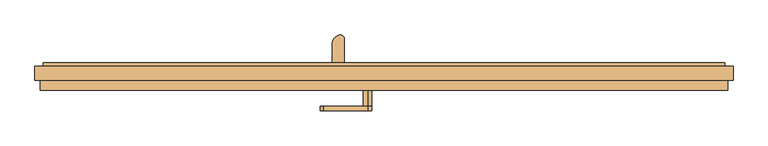
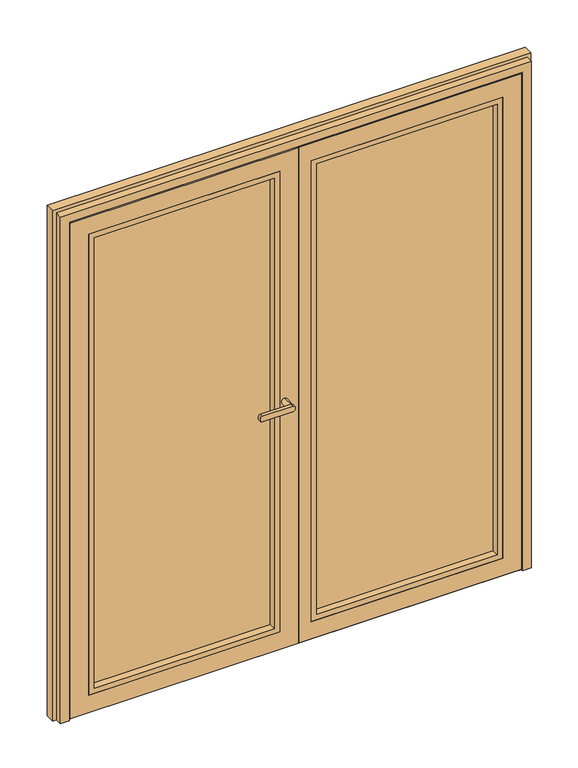
"""IFC4 building model written with IfcOpenShell, lengths in millimetres: door geometry, Schueco_FWS_ADS-75-HD-HI_inw_Family-02 : FWS SI insert unit."""

from ifc_helpers import new_model, si_unit, point, frame, frame_2d, origin, place, context, project, spatial, polyline, circle_curve, ellipse_curve, trimmed, segment, composite_curve, outline, extrude, faceted_brep, source, transform, mapped, element, save
from ifc_brep_helpers import plane_surface, cylinder_surface, extruded_surface, advanced_brep


def door_6b0dbaab(model_context):
    return source(origin(), model_context, "Body", "SolidModel", [
        faceted_brep([(900.0, -57.5000065, 8.0), (900.0, -57.5000065, 2100.0), (900.0, -66.0002823, 2100.0), (900.0, -66.0002823, 8.0), (15.0, -66.0002823, 8.0), (15.0, -57.5000065, 8.0), (15.0, -57.5000065, 23.0), (885.0, -57.5000065, 23.0), (885.0, -57.5000065, 2085.0), (15.0, -57.5000065, 2085.0), (15.0, -57.5000065, 2100.0), (15.0, -66.0002823, 2100.0), (63.0, -66.0002823, 81.0), (63.0, -66.0002823, 2027.0), (827.0, -66.0002823, 2027.0), (827.0, -66.0002823, 81.0), (827.0, 0.4997603, 2027.0), (827.0, 0.4997603, 81.0), (63.0, 0.4997603, 81.0), (63.0, 0.4997603, 2027.0), (88.0, 0.4997603, 106.0), (88.0, 0.4997603, 2002.0), (802.0, 0.4997603, 2002.0), (802.0, 0.4997603, 106.0), (802.0, 8.9997177, 2002.0), (802.0, 8.9997177, 106.0), (88.0, 8.9997177, 106.0), (88.0, 8.9997177, 2002.0), (875.0, 8.9997177, 33.0), (-10.0, 8.9997177, 33.0), (-10.0, 8.9997177, 2075.0), (875.0, 8.9997177, 2075.0), (875.0, 0.4997603, 2075.0), (875.0, 0.4997603, 33.0), (5.0, 0.4997603, 33.0), (-10.0, 0.4997603, 33.0), (5.0, 0.4997603, 23.0), (5.0, 0.4997603, 2075.0), (5.0, 0.4997603, 2085.0), (885.0, 0.4997603, 2085.0), (885.0, 0.4997603, 23.0), (5.0, -57.5000065, 23.0), (5.0, -57.5000065, 2085.0), (-10.0, 0.4997603, 2075.0)], [[[0, 1, 2, 3]], [[3, 4, 5, 0]], [[0, 5, 6, 7, 8, 9, 10, 1]], [[2, 11, 4, 3], [12, 13, 14, 15]], [[15, 14, 16, 17]], [[17, 18, 12, 15]], [[18, 19, 13, 12]], [[17, 16, 19, 18], [20, 21, 22, 23]], [[23, 22, 24, 25]], [[25, 26, 20, 23]], [[26, 27, 21, 20]], [[28, 29, 30, 31], [25, 24, 27, 26]], [[28, 31, 32, 33]], [[33, 34, 35, 29, 28]], [[36, 34, 33, 32, 37, 38, 39, 40]], [[40, 39, 8, 7]], [[7, 6, 41, 36, 40]], [[41, 42, 38, 37, 34, 36]], [[1, 10, 11, 2]], [[19, 16, 14, 13]], [[27, 24, 22, 21]], [[31, 30, 43, 37, 32]], [[42, 9, 8, 39, 38]], [[6, 5, 4, 11, 10, 9]], [[35, 43, 30, 29]], [[35, 34, 37, 43]], [[9, 42, 41, 6]]]),
        extrude(outline(polyline([(81.0, 63.0), (81.0, 827.0), (2027.0, 827.0), (2027.0, 63.0), (81.0, 63.0)]), holes=[polyline([(103.0, 805.0), (103.0, 85.0), (2005.0, 85.0), (2005.0, 805.0), (103.0, 805.0)])]), frame((0.0, -66.0002823, 0.0), z_axis=(0.0, 1.0, 0.0), x_axis=(0.0, 0.0, 1.0)), (0.0, 0.0, 1.0), 28.5000426),
        extrude(outline(polyline([(63.0, -37.5002397), (63.0, 0.4997603), (827.0, 0.4997603), (827.0, -37.5002397), (63.0, -37.5002397)])), frame((0.0, 0.0, 81.0), z_axis=(0.0, 0.0, 1.0), x_axis=(1.0, 0.0, 0.0)), (0.0, 0.0, 1.0), 1946.0),
        extrude(outline(polyline([(875.0, 0.4997603), (-10.0, 0.4997603), (-10.0, 8.9997177), (875.0, 8.9997177), (875.0, 0.4997603)])), frame((0.0, 0.0, 23.0), z_axis=(0.0, 0.0, 1.0), x_axis=(1.0, 0.0, 0.0)), (0.0, 0.0, 1.0), 10.0),
        extrude(outline(composite_curve([segment(polyline([(-141.6673236, 8.9997177), (-141.6673236, 59.1618682)]), True, "CONTINUOUS"), segment(trimmed(circle_curve(frame_2d((-114.4889059, 59.1618682)), 27.1784177), [point((-141.6673236, 59.1618682))], [point((-124.0260015, 84.6120194))], False, "CARTESIAN"), True, "CONTINUOUS"), segment(trimmed(circle_curve(frame_2d((-119.9485005, 73.7310321)), 11.6198924), [point((-124.0260015, 84.6120194))], [point((-108.3286081, 73.7310321))], False, "CARTESIAN"), True, "CONTINUOUS"), segment(polyline([(-108.3286081, 73.7310321), (-108.3286081, 8.9997177), (-141.6673236, 8.9997177)]), True, "CONTINUOUS")], self_intersect=False)), frame((0.0, 0.0, 2043.9340013), z_axis=(0.0, 0.0, 1.0), x_axis=(1.0, 0.0, 0.0)), (0.0, 0.0, 1.0), 4.0),
        extrude(outline(polyline([(-141.6673236, 12.9997177), (-108.3286081, 12.9997177), (-108.3286081, 8.9997177), (-141.6673236, 8.9997177), (-141.6673236, 12.9997177)])), frame((0.0, 0.0, 2013.9340013), z_axis=(0.0, 0.0, 1.0), x_axis=(1.0, 0.0, 0.0)), (0.0, 0.0, 1.0), 30.0),
        extrude(outline(polyline([(-141.6673236, 12.9997177), (-108.3286081, 12.9997177), (-108.3286081, 8.9997177), (-141.6673236, 8.9997177), (-141.6673236, 12.9997177)])), frame((0.0, 0.0, 56.9340013), z_axis=(0.0, 0.0, 1.0), x_axis=(1.0, 0.0, 0.0)), (0.0, 0.0, 1.0), 30.0),
        extrude(outline(composite_curve([segment(polyline([(-141.6673236, 8.9997177), (-141.6673236, 59.1618682)]), True, "CONTINUOUS"), segment(trimmed(circle_curve(frame_2d((-114.4889059, 59.1618682)), 27.1784177), [point((-141.6673236, 59.1618682))], [point((-124.0260015, 84.6120194))], False, "CARTESIAN"), True, "CONTINUOUS"), segment(trimmed(circle_curve(frame_2d((-119.9485005, 73.7310321)), 11.6198924), [point((-124.0260015, 84.6120194))], [point((-108.3286081, 73.7310321))], False, "CARTESIAN"), True, "CONTINUOUS"), segment(polyline([(-108.3286081, 73.7310321), (-108.3286081, 8.9997177), (-141.6673236, 8.9997177)]), True, "CONTINUOUS")], self_intersect=False)), frame((0.0, 0.0, 52.9340013), z_axis=(0.0, 0.0, 1.0), x_axis=(1.0, 0.0, 0.0)), (0.0, 0.0, 1.0), 4.0),
        advanced_brep(
        [(-112.282924, 57.5977179, 2043.9340013), (-137.717076, 72.2821425, 2043.9340013), (-112.282924, 57.5977179, 56.9340013), (-137.717076, 72.2821425, 56.9340013)],
        [
            (0, 1, ellipse_curve(frame((-125.0, 64.9399302, 2043.9340013), z_axis=(0.0, 0.0, 1.0000000000000002), x_axis=(0.5000002582658958, 0.866025254674503, 0.0)), 21.5840887, 14.6844171)),
            (1, 0, ellipse_curve(frame((-125.0, 64.9399302, 2043.9340013), z_axis=(0.0, 0.0, 1.0000000000000002), x_axis=(0.5000002582658958, 0.866025254674503, 0.0)), 21.5840887, 14.6844171)),
            (2, 3, ellipse_curve(frame((-125.0, 64.9399302, 56.9340013), z_axis=(0.0, 0.0, -1.0000000000000002), x_axis=(-0.866025254674503, 0.5000002582658958, 0.0)), 14.6844171, 21.5840887)),
            (3, 2, ellipse_curve(frame((-125.0, 64.9399302, 56.9340013), z_axis=(0.0, 0.0, -1.0000000000000002), x_axis=(-0.866025254674503, 0.5000002582658958, 0.0)), 14.6844171, 21.5840887)),
            (0, 2),
            (3, 1),
        ],
        [
            plane_surface(frame((-137.717076, 72.2821425, 2043.9340013), z_axis=(0.0, 0.0, 1.0000000000000002), x_axis=(0.5000002582658958, 0.866025254674503, 0.0))),
            plane_surface(frame((-137.717076, 72.2821425, 56.9340013), z_axis=(0.0, 0.0, -1.0000000000000002), x_axis=(-0.5000002582658958, -0.866025254674503, 0.0))),
            extruded_surface(trimmed(ellipse_curve(frame((-125.0, 64.9399302, 56.9340013), z_axis=(0.0, 0.0, -1.0000000000000002), x_axis=(-0.866025254674503, 0.5000002582658958, 0.0)), 14.6844171, 21.5840887), [point((-137.717076, 72.2821425, 56.9340013))], [point((-112.282924, 57.5977179, 56.9340013))], True, "CARTESIAN"), (0.0, 0.0, -1987.0), 1987.0),
            extruded_surface(trimmed(ellipse_curve(frame((-125.0, 64.9399302, 56.9340013), z_axis=(0.0, 0.0, -1.0000000000000002), x_axis=(-0.866025254674503, 0.5000002582658958, 0.0)), 14.6844171, 21.5840887), [point((-112.282924, 57.5977179, 56.9340013))], [point((-137.717076, 72.2821425, 56.9340013))], True, "CARTESIAN"), (0.0, 0.0, -1987.0), 1987.0),
        ],
        [
            (0, [[1, 2]]),
            (1, [[3, 4]]),
            (2, [[5, -4, 6, -1]]),
            (3, [[-6, -3, -5, -2]]),
        ],
    ),
        advanced_brep(
        [(-45.0, -122.0002518, 1038.0113692), (-45.0, -122.0002518, 1061.9886308), (-166.6617926, -122.0002518, 1061.9886308), (-166.6617926, -122.0002518, 1038.0113692), (-45.0, -109.5001648, 1061.9886308), (-45.0, -109.5001648, 1038.0113692), (-166.6617926, -109.5001648, 1038.0113692), (-166.6617926, -109.5001648, 1061.9886308), (-45.0, -66.0002823, 1038.0113692), (-45.0, -66.0002823, 1061.9886308)],
        [
            (0, 1, circle_curve(frame((-45.0, -122.0002518, 1050.0), z_axis=(0.0, -1.0, 0.0), x_axis=(0.0, 0.0, 1.0)), 11.9886308)),
            (1, 2),
            (2, 3, ellipse_curve(frame((-166.6617926, -122.0002518, 1050.0), z_axis=(0.0, -1.0, 0.0), x_axis=(0.0, 0.0, -1.0)), 11.9886308, 7.9050795)),
            (3, 0),
            (4, 5, circle_curve(frame((-45.0, -109.5001648, 1050.0), z_axis=(0.0, -1.0, 0.0), x_axis=(0.0, 0.0, 1.0)), 11.9886308)),
            (5, 6),
            (6, 7, ellipse_curve(frame((-166.6617926, -109.5001648, 1050.0), z_axis=(0.0, 1.0, 0.0), x_axis=(0.0, 0.0, -1.0)), 11.9886308, 7.9050795)),
            (7, 4),
            (3, 6),
            (5, 0),
            (2, 7),
            (1, 4),
            (5, 4, circle_curve(frame((-45.0, -109.5001648, 1050.0), z_axis=(0.0, -1.0, 0.0), x_axis=(0.0, 0.0, 1.0)), 11.9886308)),
            (8, 9, circle_curve(frame((-45.0, -66.0002823, 1050.0), z_axis=(0.0, 1.0, 0.0), x_axis=(0.0, 0.0, 1.0)), 11.9886308)),
            (9, 8, circle_curve(frame((-45.0, -66.0002823, 1050.0), z_axis=(0.0, 1.0, 0.0), x_axis=(0.0, 0.0, 1.0)), 11.9886308)),
            (8, 5),
            (4, 9),
        ],
        [
            plane_surface(frame((-166.6617926, -122.0002518, 1038.0113692), z_axis=(0.0, -1.0, 0.0), x_axis=(-1.0, 0.0, 0.0))),
            plane_surface(frame((-166.6617926, -109.5001648, 1038.0113692), z_axis=(0.0, 1.0, 0.0), x_axis=(1.0, 0.0, 0.0))),
            plane_surface(frame((-45.0, -122.0002518, 1038.0113692), z_axis=(0.0, 0.0, -1.0), x_axis=(0.0, 1.0, 0.0))),
            extruded_surface(trimmed(ellipse_curve(frame((-166.6617926, -109.5001648, 1050.0), z_axis=(0.0, 1.0, 0.0), x_axis=(0.0, 0.0, -1.0)), 11.9886308, 7.9050795), [point((-166.6617926, -109.5001648, 1038.0113692))], [point((-166.6617926, -109.5001648, 1061.9886308))], True, "CARTESIAN"), (0.0, 12.500086999999994, 0.0), 12.500086999999994),
            plane_surface(frame((-166.6617926, -122.0002518, 1061.9886308), z_axis=(0.0, 0.0, 1.0), x_axis=(0.0, 1.0, 0.0))),
            cylinder_surface(frame((-45.0, -109.5001648, 1050.0), z_axis=(0.0, -1.0, 0.0), x_axis=(0.0, 0.0, 1.0)), 11.9886308),
            plane_surface(frame((-45.0, -66.0002823, 1061.9886308), z_axis=(0.0, 1.0, 0.0), x_axis=(-1.0, 0.0, 0.0))),
            cylinder_surface(frame((-45.0, -66.0002823, 1050.0), z_axis=(0.0, -1.0, 0.0), x_axis=(0.0, 0.0, 1.0)), 11.9886308),
        ],
        [
            (0, [[1, 2, 3, 4]]),
            (1, [[5, 6, 7, 8]]),
            (2, [[9, -6, 10, -4]]),
            (3, [[11, -7, -9, -3]]),
            (4, [[12, -8, -11, -2]]),
            (5, [[-10, 13, -12, -1]]),
            (6, [[14, 15]]),
            (7, [[16, -5, 17, -14]]),
            (7, [[-17, -13, -16, -15]]),
        ],
    ),
        faceted_brep([(-900.0, -57.5000065, 8.0), (-900.0, -66.0002823, 8.0), (-900.0, -66.0002823, 2100.0), (-900.0, -57.5000065, 2100.0), (10.0, -57.5000065, 8.0), (10.0, -66.0002823, 8.0), (10.0, -57.5000065, 2100.0), (-885.0, -57.5000065, 23.0), (-5.0, -57.5000065, 23.0), (-5.0, -57.5000065, 2085.0), (-885.0, -57.5000065, 2085.0), (10.0, -66.0002823, 2100.0), (-63.0, -66.0002823, 81.0), (-827.0, -66.0002823, 81.0), (-827.0, -66.0002823, 2027.0), (-63.0, -66.0002823, 2027.0), (-827.0, 0.4997603, 81.0), (-827.0, 0.4997603, 2027.0), (-63.0, 0.4997603, 81.0), (-63.0, 0.4997603, 2027.0), (-88.0, 0.4997603, 106.0), (-802.0, 0.4997603, 106.0), (-802.0, 0.4997603, 2002.0), (-88.0, 0.4997603, 2002.0), (-802.0, 8.9997177, 106.0), (-802.0, 8.9997177, 2002.0), (-88.0, 8.9997177, 106.0), (-88.0, 8.9997177, 2002.0), (-15.0, 8.9997177, 2075.0), (-15.0, 8.9997177, 33.0), (-25.0, 8.9997177, 33.0), (-875.0, 8.9997177, 33.0), (-875.0, 8.9997177, 2075.0), (-25.0, 8.9997177, 2075.0), (-875.0, 0.4997603, 33.0), (-875.0, 0.4997603, 2075.0), (-15.0, 0.4997603, 33.0), (-25.0, 0.4997603, 33.0), (-15.0, 0.4997603, 2075.0), (-5.0, 0.4997603, 23.0), (-885.0, 0.4997603, 23.0), (-885.0, 0.4997603, 2085.0), (-5.0, 0.4997603, 2085.0), (-25.0, 0.4997603, 2075.0)], [[[0, 1, 2, 3]], [[1, 0, 4, 5]], [[4, 0, 3, 6], [7, 8, 9, 10]], [[5, 4, 6, 11]], [[1, 5, 11, 2], [12, 13, 14, 15]], [[13, 16, 17, 14]], [[16, 13, 12, 18]], [[18, 12, 15, 19]], [[16, 18, 19, 17], [20, 21, 22, 23]], [[21, 24, 25, 22]], [[24, 21, 20, 26]], [[26, 20, 23, 27]], [[28, 29, 30, 31, 32, 33], [24, 26, 27, 25]], [[31, 34, 35, 32]], [[34, 31, 30, 29, 36, 37]], [[36, 29, 28, 38]], [[39, 40, 41, 42], [36, 38, 43, 35, 34, 37]], [[40, 7, 10, 41]], [[7, 40, 39, 8]], [[8, 39, 42, 9]], [[11, 6, 3, 2]], [[19, 15, 14, 17]], [[27, 23, 22, 25]], [[38, 28, 33, 32, 35, 43]], [[9, 42, 41, 10]]]),
        extrude(outline(polyline([(81.0, -63.0), (2027.0, -63.0), (2027.0, -827.0), (81.0, -827.0), (81.0, -63.0)]), holes=[polyline([(103.0, -805.0), (2005.0, -805.0), (2005.0, -85.0), (103.0, -85.0), (103.0, -805.0)])]), frame((0.0, -66.0002823, 0.0), z_axis=(0.0, 1.0, 0.0), x_axis=(0.0, 0.0, 1.0)), (0.0, 0.0, 1.0), 28.5000426),
        extrude(outline(polyline([(-63.0, -37.5002397), (-827.0, -37.5002397), (-827.0, 0.4997603), (-63.0, 0.4997603), (-63.0, -37.5002397)])), frame((0.0, 0.0, 81.0), z_axis=(0.0, 0.0, 1.0), x_axis=(1.0, 0.0, 0.0)), (0.0, 0.0, 1.0), 1946.0),
        extrude(outline(polyline([(-875.0, 0.4997603), (-875.0, 8.9997177), (-15.0, 8.9997177), (-15.0, 0.4997603), (-875.0, 0.4997603)])), frame((0.0, 0.0, 23.0), z_axis=(0.0, 0.0, 1.0), x_axis=(1.0, 0.0, 0.0)), (0.0, 0.0, 1.0), 10.0),
        faceted_brep([(930.999943, 8.9997177, 2130.999943), (930.999943, 0.0, 2130.999943), (930.999943, 0.0, 0.0), (930.999943, 8.9997177, 0.0), (-954.0, 0.0, 0.0), (-954.0, 0.0, 2154.0), (954.0, 0.0, 2154.0), (954.0, 0.0, 0.0), (-930.999943, 0.0, 2130.999943), (-930.999943, 0.0, 0.0), (954.0, -38.0, 0.0), (940.0, -38.0, 0.0), (940.0, -66.0002823, 0.0), (904.9999114, -66.0002823, 0.0), (904.9999114, -57.5000065, 0.0), (893.4999114, -57.5000065, 0.0), (893.4999114, 0.4997603, 0.0), (879.9999888, 0.4997603, 0.0), (879.9999888, 8.9997177, 0.0), (-879.9999888, 8.9997177, 0.0), (-930.999943, 8.9997177, 0.0), (-930.999943, 8.9997177, 2130.999943), (879.9999888, 8.9997177, 2079.9999888), (-879.9999888, 8.9997177, 2079.9999888), (904.9999114, -66.0002823, 2104.9999114), (904.9999114, -57.5000065, 2104.9999114), (-904.9999114, -57.5000065, 0.0), (-893.4999114, -57.5000065, 0.0), (-893.4999114, -57.5000065, 2093.4999114), (893.4999114, -57.5000065, 2093.4999114), (-904.9999114, -57.5000065, 2104.9999114), (-940.0, -66.0002823, 0.0), (-904.9999114, -66.0002823, 0.0), (-904.9999114, -66.0002823, 2104.9999114), (940.0, -66.0002823, 2140.0), (-940.0, -66.0002823, 2140.0), (940.0, -38.0, 2140.0), (-954.0, -38.0, 0.0), (-940.0, -38.0, 0.0), (-940.0, -38.0, 2140.0), (954.0, -38.0, 2154.0), (-954.0, -38.0, 2154.0), (-879.9999888, 0.4997603, 0.0), (-893.4999114, 0.4997603, 0.0), (879.9999888, 0.4997603, 2079.9999888), (-879.9999888, 0.4997603, 2079.9999888), (893.4999114, 0.4997603, 2093.4999114), (-893.4999114, 0.4997603, 2093.4999114)], [[[0, 1, 2, 3]], [[4, 5, 6, 7, 2, 1, 8, 9]], [[3, 2, 7, 10, 11, 12, 13, 14, 15, 16, 17, 18]], [[19, 20, 21, 0, 3, 18, 22, 23]], [[24, 25, 14, 13]], [[26, 27, 28, 29, 15, 14, 25, 30]], [[31, 32, 33, 24, 13, 12, 34, 35]], [[34, 12, 11, 36]], [[37, 38, 39, 36, 11, 10, 40, 41]], [[4, 9, 20, 19, 42, 43, 27, 26, 32, 31, 38, 37]], [[20, 9, 8, 21]], [[18, 17, 44, 22]], [[42, 19, 23, 45]], [[32, 26, 30, 33]], [[31, 35, 39, 38]], [[4, 37, 41, 5]], [[6, 40, 10, 7]], [[43, 42, 45, 44, 17, 16, 46, 47]], [[16, 15, 29, 46]], [[27, 43, 47, 28]], [[21, 8, 1, 0]], [[33, 30, 25, 24]], [[35, 34, 36, 39]], [[23, 22, 44, 45]], [[5, 41, 40, 6]], [[47, 46, 29, 28]]]),
        extrude(outline(polyline([(8.9997177, 12.6266542), (8.9997177, 0.0), (-57.5000065, 0.0), (-57.5000065, 14.9999981), (-13.699618, 14.9999981), (-8.699618, 19.9999981), (-6.8140015, 19.9999981), (8.9997177, 12.6266542)])), frame((-895.5, 0.0, 0.0), z_axis=(1.0, 0.0, 0.0), x_axis=(0.0, 1.0, 0.0)), (0.0, 0.0, 1.0), 1790.9999732),
    ])


if __name__ == "__main__":
    model = new_model("IFC4")
    model_context = context("Model", 3, world=origin())
    ifc_project = project(units=[si_unit("LENGTHUNIT", "METRE", prefix="MILLI")], contexts=[model_context])
    site = spatial("IfcSite", under=ifc_project)
    building = spatial("IfcBuilding", under=site)
    placement = place(None, origin())
    door_shape = door_6b0dbaab(model_context)
    element("IfcDoor", 1, ObjectType="Schueco_FWS_ADS-75-HD-HI_inw_Family-02 : FWS SI insert unit", at=placement, inside=building, context=model_context, shape_type="MappedRepresentation", body=[
        mapped(door_shape, transform((0.0, 0.0, 0.0), x_axis=(1.0, 0.0, 0.0), y_axis=(0.0, 1.0, 0.0), z_axis=(0.0, 0.0, 1.0))),
    ])
    save(model, "model.ifc")

# Revit data of these elements
# Type "Schueco_FWS_ADS-75-HD-HI_inw_Family-02 : FWS SI insert unit"
#   Type Mark = "48"
#   __NOTE__ = "Data describes the optimum values of the entire system. The properites of a selected design option have to be determined on an individual basis!"
#   Wind load resistance = "Class 2"
#   Watertightness = "Class 5A"
#   Thermal insulation = "Uf = 1.4 W/(m²K)"
#   Sound insulation = "Rw 43 dB"
#   Schueco thermal insulation standard = "Highly thermally insulated"
#   Opening type = "Inward-opening, Flush-fitted"
#   Model = "Schueco ADS 75 HD.HI"
#   Mechanical loading = "Class 2"
#   Maximum leaf width in mm = "1400"
#   Maximum leaf weight in kg = "200"
#   Maximum leaf height in mm = "3000"
#   Material = "Aluminium"
#   Long term functionality = "Class 6"
#   Construction Type = "Door, double-leaf, inward-opening"
#   Manufacturer = "Schueco International KG"
#   Glazing data = "Triple glazing 38mm"
#   Façade insert unit = "yes"
#   Family creation date = "08.2017"
#   Description = "Schueco Aluminium Door System (ADS)"
#   Burglar resistance = "Class RC 3"
#   Areas of use = "Public buildings"
#   Analytic Construction = "<None>"
#   Air permeability = "Class 2"
#   Width [instance default] = 1709.145 mm
#   Leaf opening angle [instance default] = 0.00°
#   IOf_T = 38 mm
#   Height [instance default] = 2117.739 mm
#   Glazing area [instance default] = 2.28589 m²
#   F2_W [instance default] = 854.572 mm
#   F1_W [instance default] = 854.572 mm
#   Distance from bottom to handles [instance default] = 1050 mm
#   Clear opening width [instance default] = 1561.145 mm
#   Active leaf width = 1100 mm
#   Standard threshold = yes
#   Low level threshold = no
#   Handles = yes
#   FWS SI insert unit = yes
#   FWS HI insert unit = no
#   All fields of identical width = yes
#   Glass = none
#   Frame = Alu
#   Fittings = none
# Element 1 (IfcDoor, "Schueco_FWS_ADS-75-HD-HI_inw_Family-02 : FWS SI insert unit")
#   Width = 1908 mm
#   Height = 2154 mm
#   Glazing area = 2.70749 m²
#   F2_W = 954 mm
#   F1_W = 954 mm
#   Clear opening width = 1760 mm
#   Materials on its faces: "Alu", "Glass"
# Materials
#   "Alu": class "Glas", colour RGB 140 140 140, transparency 0
#   "Glass": class "Glass", colour RGB 128 128 255, transparency 0.75, Description = "Soda Lime Glass", Cost = 0
